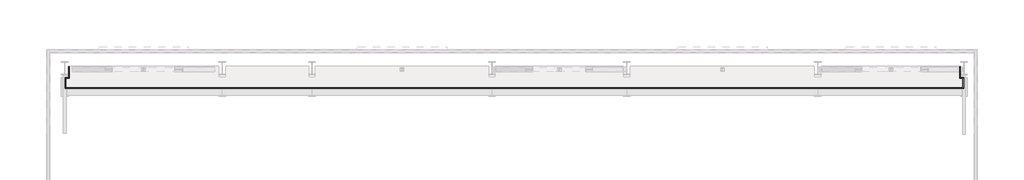
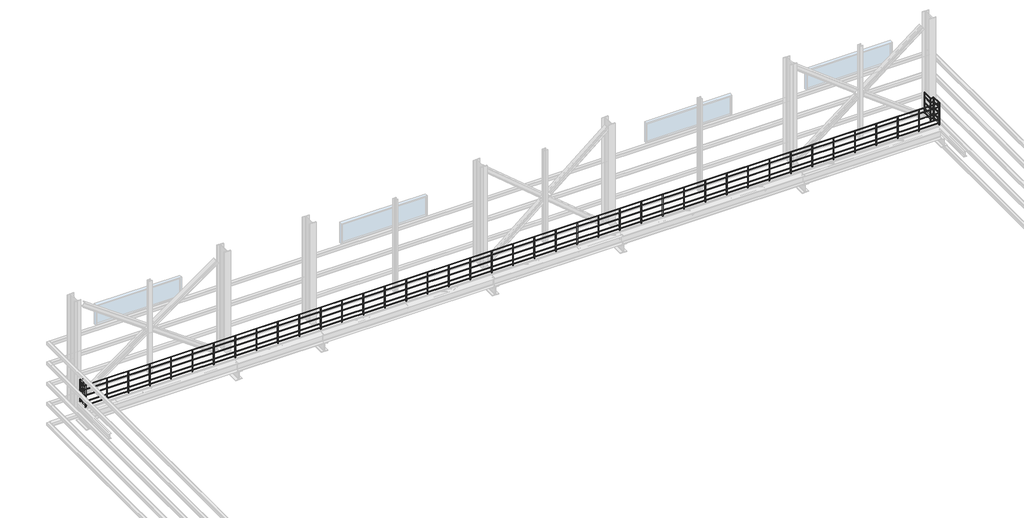
# One storey, part 4 of 4: 1 railing.
"""IFC4 building model written with IfcOpenShell, lengths in millimetres."""

from ifc_helpers import new_model, si_unit, frame, origin, place, context, project, spatial, polyline, circle_curve, ellipse_curve, outline, extrude, element, save
from ifc_brep_helpers import plane_surface, cylinder_surface, advanced_brep

model = new_model("IFC4")

# Units and contexts
model_context = context("Model", 3, world=origin())
ifc_project = project(units=[si_unit("LENGTHUNIT", "METRE", prefix="MILLI")], contexts=[model_context])

# Site, building, storey
site = spatial("IfcSite", under=ifc_project)
building = spatial("IfcBuilding", under=site)
storey = spatial("IfcBuildingStorey", under=building, Name="T.O.CRANE GIR.", Elevation=12299.9720055)

# Railing
placement = place(None, origin())
element("IfcRailing", 1, ObjectType="H_RL_AMH_Steel Handrail_H1100", at=placement, inside=storey, context=model_context, shape_type="SolidModel", body=[
    advanced_brep(
    [(165.0, 39119.5208589, 13466.9720055), (195.0, 39119.5208589, 13466.9720055), (165.0, 38634.5208589, 13466.9720055), (195.0, 38604.5208589, 13466.9720055), (15.0, 38634.5208589, 13466.9720055), (45.0, 38604.5208589, 13466.9720055), (15.0, 38164.5208589, 13466.9720055), (45.0, 38194.5208589, 13466.9720055), (39985.0, 38164.5208589, 13466.9720055), (39955.0, 38194.5208589, 13466.9720055), (39985.0, 38634.5208589, 13466.9720055), (39955.0, 38604.5208589, 13466.9720055), (39835.0, 38634.5208589, 13466.9720055), (39805.0, 38604.5208589, 13466.9720055), (39835.0, 39119.5208589, 13466.9720055), (39805.0, 39119.5208589, 13466.9720055)],
    [
        (0, 1, circle_curve(frame((180.0, 39119.5208589, 13466.9720055), z_axis=(0.0, 1.0, 0.0), x_axis=(1.0, 0.0, 0.0)), 15.0)),
        (1, 0, circle_curve(frame((180.0, 39119.5208589, 13466.9720055), z_axis=(0.0, 1.0, 0.0), x_axis=(1.0, 0.0, 0.0)), 15.0)),
        (0, 2),
        (2, 3, ellipse_curve(frame((180.0, 38619.5208589, 13466.9720055), z_axis=(0.707106781186548, 0.7071067811865469, 0.0), x_axis=(-0.7071067811865468, 0.7071067811865482, 0.0)), 21.2132034, 15.0)),
        (3, 1),
        (3, 2, ellipse_curve(frame((180.0, 38619.5208589, 13466.9720055), z_axis=(0.707106781186548, 0.7071067811865469, 0.0), x_axis=(-0.7071067811865468, 0.7071067811865482, 0.0)), 21.2132034, 15.0)),
        (2, 4),
        (4, 5, ellipse_curve(frame((30.0, 38619.5208589, 13466.9720055), z_axis=(0.707106781186548, 0.7071067811865469, 0.0), x_axis=(0.7071067811865472, -0.7071067811865479, 0.0)), 21.2132034, 15.0)),
        (5, 3),
        (5, 4, ellipse_curve(frame((30.0, 38619.5208589, 13466.9720055), z_axis=(0.707106781186548, 0.7071067811865469, 0.0), x_axis=(0.7071067811865472, -0.7071067811865479, 0.0)), 21.2132034, 15.0)),
        (4, 6),
        (6, 7, ellipse_curve(frame((30.0, 38179.5208589, 13466.9720055), z_axis=(-0.7071067811865459, 0.7071067811865491, 0.0), x_axis=(0.7071067811865491, 0.7071067811865458, 0.0)), 21.2132034, 15.0)),
        (7, 5),
        (7, 6, ellipse_curve(frame((30.0, 38179.5208589, 13466.9720055), z_axis=(-0.7071067811865459, 0.7071067811865491, 0.0), x_axis=(0.7071067811865491, 0.7071067811865458, 0.0)), 21.2132034, 15.0)),
        (6, 8),
        (8, 9, ellipse_curve(frame((39970.0, 38179.5208589, 13466.9720055), z_axis=(-0.7071067811865486, -0.7071067811865465, 0.0), x_axis=(-0.7071067811865465, 0.7071067811865486, 0.0)), 21.2132034, 15.0)),
        (9, 7),
        (9, 8, ellipse_curve(frame((39970.0, 38179.5208589, 13466.9720055), z_axis=(-0.7071067811865486, -0.7071067811865465, 0.0), x_axis=(-0.7071067811865465, 0.7071067811865486, 0.0)), 21.2132034, 15.0)),
        (8, 10),
        (10, 11, ellipse_curve(frame((39970.0, 38619.5208589, 13466.9720055), z_axis=(0.7071067811865476, -0.7071067811865474, 0.0), x_axis=(-0.7071067811865472, -0.7071067811865478, 0.0)), 21.2132034, 15.0)),
        (11, 9),
        (11, 10, ellipse_curve(frame((39970.0, 38619.5208589, 13466.9720055), z_axis=(0.7071067811865476, -0.7071067811865474, 0.0), x_axis=(-0.7071067811865472, -0.7071067811865478, 0.0)), 21.2132034, 15.0)),
        (10, 12),
        (12, 13, ellipse_curve(frame((39820.0, 38619.5208589, 13466.9720055), z_axis=(0.7071067811865476, -0.7071067811865474, 0.0), x_axis=(0.7071067811865475, 0.7071067811865475, 0.0)), 21.2132034, 15.0)),
        (13, 11),
        (13, 12, ellipse_curve(frame((39820.0, 38619.5208589, 13466.9720055), z_axis=(0.7071067811865476, -0.7071067811865474, 0.0), x_axis=(0.7071067811865475, 0.7071067811865475, 0.0)), 21.2132034, 15.0)),
        (14, 15, circle_curve(frame((39820.0, 39119.5208589, 13466.9720055), z_axis=(0.0, 1.0, 0.0), x_axis=(-1.0, 0.0, 0.0)), 15.0)),
        (15, 14, circle_curve(frame((39820.0, 39119.5208589, 13466.9720055), z_axis=(0.0, 1.0, 0.0), x_axis=(-1.0, 0.0, 0.0)), 15.0)),
        (12, 14),
        (15, 13),
    ],
    [
        plane_surface(frame((180.0, 39119.5208589, 13481.9720055), z_axis=(0.0, 1.0, 0.0), x_axis=(0.0, 0.0, -1.0))),
        cylinder_surface(frame((180.0, 39119.5208589, 13466.9720055), z_axis=(0.0, 1.0, 0.0), x_axis=(1.0, 0.0, 0.0)), 15.0),
        cylinder_surface(frame((180.0, 38619.5208589, 13466.9720055), z_axis=(1.0, 0.0, 0.0), x_axis=(0.0, -1.0, 0.0)), 15.0),
        cylinder_surface(frame((30.0, 38619.5208589, 13466.9720055), z_axis=(0.0, 1.0, 0.0), x_axis=(1.0, 0.0, 0.0)), 15.0),
        cylinder_surface(frame((30.0, 38179.5208589, 13466.9720055), z_axis=(-1.0, 0.0, 0.0), x_axis=(0.0, 1.0, 0.0)), 15.0),
        cylinder_surface(frame((39970.0, 38179.5208589, 13466.9720055), z_axis=(0.0, -1.0, 0.0), x_axis=(-1.0, 0.0, 0.0)), 15.0),
        cylinder_surface(frame((39970.0, 38619.5208589, 13466.9720055), z_axis=(1.0, 0.0, 0.0), x_axis=(0.0, -1.0, 0.0)), 15.0),
        plane_surface(frame((39820.0, 39119.5208589, 13481.9720055), z_axis=(0.0, 1.0, 0.0), x_axis=(0.0, 0.0, 1.0))),
        cylinder_surface(frame((39820.0, 38619.5208589, 13466.9720055), z_axis=(0.0, -1.0, 0.0), x_axis=(-1.0, 0.0, 0.0)), 15.0),
    ],
    [
        (0, [[1, 2]]),
        (1, [[-1, 3, 4, 5]]),
        (1, [[-2, -5, 6, -3]]),
        (2, [[-4, 7, 8, 9]]),
        (2, [[-6, -9, 10, -7]]),
        (3, [[-8, 11, 12, 13]]),
        (3, [[-10, -13, 14, -11]]),
        (4, [[-12, 15, 16, 17]]),
        (4, [[-14, -17, 18, -15]]),
        (5, [[-16, 19, 20, 21]]),
        (5, [[-18, -21, 22, -19]]),
        (6, [[-20, 23, 24, 25]]),
        (6, [[-22, -25, 26, -23]]),
        (7, [[27, 28]]),
        (8, [[-24, 29, -28, 30]]),
        (8, [[-26, -30, -27, -29]]),
    ],
),
    advanced_brep(
    [(15.0, 38634.5208589, 13266.9720055), (45.0, 38604.5208589, 13266.9720055), (45.0, 38194.5208589, 13266.9720055), (15.0, 38164.5208589, 13266.9720055), (39955.0, 38194.5208589, 13266.9720055), (39985.0, 38164.5208589, 13266.9720055), (39955.0, 38604.5208589, 13266.9720055), (39985.0, 38634.5208589, 13266.9720055), (39805.0, 38604.5208589, 13266.9720055), (39835.0, 38634.5208589, 13266.9720055), (39805.0, 39119.5208589, 13266.9720055), (39835.0, 39119.5208589, 13266.9720055), (195.0, 39119.5208589, 13266.9720055), (165.0, 39119.5208589, 13266.9720055), (195.0, 38604.5208589, 13266.9720055), (165.0, 38634.5208589, 13266.9720055)],
    [
        (0, 1, ellipse_curve(frame((30.0, 38619.5208589, 13266.9720055), z_axis=(-0.707106781186548, -0.7071067811865469, 0.0), x_axis=(-0.7071067811865467, 0.7071067811865482, 0.0)), 21.2132034, 15.0)),
        (1, 2),
        (2, 3, ellipse_curve(frame((30.0, 38179.5208589, 13266.9720055), z_axis=(-0.7071067811865459, 0.7071067811865491, 0.0), x_axis=(0.7071067811865491, 0.7071067811865458, 0.0)), 21.2132034, 15.0)),
        (3, 0),
        (1, 0, ellipse_curve(frame((30.0, 38619.5208589, 13266.9720055), z_axis=(-0.707106781186548, -0.7071067811865469, 0.0), x_axis=(-0.7071067811865467, 0.7071067811865482, 0.0)), 21.2132034, 15.0)),
        (3, 2, ellipse_curve(frame((30.0, 38179.5208589, 13266.9720055), z_axis=(-0.7071067811865459, 0.7071067811865491, 0.0), x_axis=(0.7071067811865491, 0.7071067811865458, 0.0)), 21.2132034, 15.0)),
        (2, 4),
        (4, 5, ellipse_curve(frame((39970.0, 38179.5208589, 13266.9720055), z_axis=(-0.7071067811865486, -0.7071067811865465, 0.0), x_axis=(-0.7071067811865465, 0.7071067811865486, 0.0)), 21.2132034, 15.0)),
        (5, 3),
        (5, 4, ellipse_curve(frame((39970.0, 38179.5208589, 13266.9720055), z_axis=(-0.7071067811865486, -0.7071067811865465, 0.0), x_axis=(-0.7071067811865465, 0.7071067811865486, 0.0)), 21.2132034, 15.0)),
        (4, 6),
        (6, 7, ellipse_curve(frame((39970.0, 38619.5208589, 13266.9720055), z_axis=(0.7071067811865476, -0.7071067811865474, 0.0), x_axis=(-0.7071067811865472, -0.7071067811865478, 0.0)), 21.2132034, 15.0)),
        (7, 5),
        (7, 6, ellipse_curve(frame((39970.0, 38619.5208589, 13266.9720055), z_axis=(0.7071067811865476, -0.7071067811865474, 0.0), x_axis=(-0.7071067811865472, -0.7071067811865478, 0.0)), 21.2132034, 15.0)),
        (6, 8),
        (8, 9, ellipse_curve(frame((39820.0, 38619.5208589, 13266.9720055), z_axis=(0.7071067811865476, -0.7071067811865474, 0.0), x_axis=(0.7071067811865475, 0.7071067811865475, 0.0)), 21.2132034, 15.0)),
        (9, 7),
        (9, 8, ellipse_curve(frame((39820.0, 38619.5208589, 13266.9720055), z_axis=(0.7071067811865476, -0.7071067811865474, 0.0), x_axis=(0.7071067811865475, 0.7071067811865475, 0.0)), 21.2132034, 15.0)),
        (10, 11, circle_curve(frame((39820.0, 39119.5208589, 13266.9720055), z_axis=(0.0, 1.0, 0.0), x_axis=(1.0, 0.0, 0.0)), 15.0)),
        (11, 10, circle_curve(frame((39820.0, 39119.5208589, 13266.9720055), z_axis=(0.0, 1.0, 0.0), x_axis=(1.0, 0.0, 0.0)), 15.0)),
        (8, 10),
        (11, 9),
        (12, 13, circle_curve(frame((180.0, 39119.5208589, 13266.9720055), z_axis=(0.0, 1.0, 0.0), x_axis=(-1.0, 0.0, 0.0)), 15.0)),
        (13, 12, circle_curve(frame((180.0, 39119.5208589, 13266.9720055), z_axis=(0.0, 1.0, 0.0), x_axis=(-1.0, 0.0, 0.0)), 15.0)),
        (12, 14),
        (14, 15, ellipse_curve(frame((180.0, 38619.5208589, 13266.9720055), z_axis=(0.707106781186548, 0.7071067811865469, 0.0), x_axis=(-0.7071067811865468, 0.7071067811865482, 0.0)), 21.2132034, 15.0)),
        (15, 13),
        (15, 14, ellipse_curve(frame((180.0, 38619.5208589, 13266.9720055), z_axis=(0.707106781186548, 0.7071067811865469, 0.0), x_axis=(-0.7071067811865468, 0.7071067811865482, 0.0)), 21.2132034, 15.0)),
        (14, 1),
        (0, 15),
    ],
    [
        cylinder_surface(frame((30.0, 38619.5208589, 13266.9720055), z_axis=(0.0, 1.0, 0.0), x_axis=(-1.0, 0.0, 0.0)), 15.0),
        cylinder_surface(frame((30.0, 38179.5208589, 13266.9720055), z_axis=(-1.0, 0.0, 0.0), x_axis=(0.0, -1.0, 0.0)), 15.0),
        cylinder_surface(frame((39970.0, 38179.5208589, 13266.9720055), z_axis=(0.0, -1.0, 0.0), x_axis=(1.0, 0.0, 0.0)), 15.0),
        cylinder_surface(frame((39970.0, 38619.5208589, 13266.9720055), z_axis=(1.0, 0.0, 0.0), x_axis=(0.0, 1.0, 0.0)), 15.0),
        plane_surface(frame((39820.0, 39119.5208589, 13281.9720055), z_axis=(0.0, 1.0, 0.0), x_axis=(0.0, 0.0, 1.0))),
        cylinder_surface(frame((39820.0, 38619.5208589, 13266.9720055), z_axis=(0.0, -1.0, 0.0), x_axis=(1.0, 0.0, 0.0)), 15.0),
        plane_surface(frame((180.0, 39119.5208589, 13281.9720055), z_axis=(0.0, 1.0, 0.0), x_axis=(0.0, 0.0, -1.0))),
        cylinder_surface(frame((180.0, 39119.5208589, 13266.9720055), z_axis=(0.0, 1.0, 0.0), x_axis=(-1.0, 0.0, 0.0)), 15.0),
        cylinder_surface(frame((180.0, 38619.5208589, 13266.9720055), z_axis=(1.0, 0.0, 0.0), x_axis=(0.0, 1.0, 0.0)), 15.0),
    ],
    [
        (0, [[1, 2, 3, 4]]),
        (0, [[5, -4, 6, -2]]),
        (1, [[-3, 7, 8, 9]]),
        (1, [[-6, -9, 10, -7]]),
        (2, [[-8, 11, 12, 13]]),
        (2, [[-10, -13, 14, -11]]),
        (3, [[-12, 15, 16, 17]]),
        (3, [[-14, -17, 18, -15]]),
        (4, [[19, 20]]),
        (5, [[-16, 21, -20, 22]]),
        (5, [[-18, -22, -19, -21]]),
        (6, [[23, 24]]),
        (7, [[-23, 25, 26, 27]]),
        (7, [[-24, -27, 28, -25]]),
        (8, [[-26, 29, -1, 30]]),
        (8, [[-28, -30, -5, -29]]),
    ],
),
    advanced_brep(
    [(15.0, 38634.5208589, 12966.9720055), (45.0, 38604.5208589, 12966.9720055), (45.0, 38194.5208589, 12966.9720055), (15.0, 38164.5208589, 12966.9720055), (39955.0, 38194.5208589, 12966.9720055), (39985.0, 38164.5208589, 12966.9720055), (39955.0, 38604.5208589, 12966.9720055), (39985.0, 38634.5208589, 12966.9720055), (39805.0, 38604.5208589, 12966.9720055), (39835.0, 38634.5208589, 12966.9720055), (39805.0, 39119.5208589, 12966.9720055), (39835.0, 39119.5208589, 12966.9720055), (195.0, 39119.5208589, 12966.9720055), (165.0, 39119.5208589, 12966.9720055), (195.0, 38604.5208589, 12966.9720055), (165.0, 38634.5208589, 12966.9720055)],
    [
        (0, 1, ellipse_curve(frame((30.0, 38619.5208589, 12966.9720055), z_axis=(-0.707106781186548, -0.7071067811865469, 0.0), x_axis=(-0.7071067811865467, 0.7071067811865482, 0.0)), 21.2132034, 15.0)),
        (1, 2),
        (2, 3, ellipse_curve(frame((30.0, 38179.5208589, 12966.9720055), z_axis=(-0.7071067811865459, 0.7071067811865491, 0.0), x_axis=(0.7071067811865491, 0.7071067811865458, 0.0)), 21.2132034, 15.0)),
        (3, 0),
        (1, 0, ellipse_curve(frame((30.0, 38619.5208589, 12966.9720055), z_axis=(-0.707106781186548, -0.7071067811865469, 0.0), x_axis=(-0.7071067811865467, 0.7071067811865482, 0.0)), 21.2132034, 15.0)),
        (3, 2, ellipse_curve(frame((30.0, 38179.5208589, 12966.9720055), z_axis=(-0.7071067811865459, 0.7071067811865491, 0.0), x_axis=(0.7071067811865491, 0.7071067811865458, 0.0)), 21.2132034, 15.0)),
        (2, 4),
        (4, 5, ellipse_curve(frame((39970.0, 38179.5208589, 12966.9720055), z_axis=(-0.7071067811865486, -0.7071067811865465, 0.0), x_axis=(-0.7071067811865465, 0.7071067811865486, 0.0)), 21.2132034, 15.0)),
        (5, 3),
        (5, 4, ellipse_curve(frame((39970.0, 38179.5208589, 12966.9720055), z_axis=(-0.7071067811865486, -0.7071067811865465, 0.0), x_axis=(-0.7071067811865465, 0.7071067811865486, 0.0)), 21.2132034, 15.0)),
        (4, 6),
        (6, 7, ellipse_curve(frame((39970.0, 38619.5208589, 12966.9720055), z_axis=(0.7071067811865476, -0.7071067811865474, 0.0), x_axis=(-0.7071067811865472, -0.7071067811865478, 0.0)), 21.2132034, 15.0)),
        (7, 5),
        (7, 6, ellipse_curve(frame((39970.0, 38619.5208589, 12966.9720055), z_axis=(0.7071067811865476, -0.7071067811865474, 0.0), x_axis=(-0.7071067811865472, -0.7071067811865478, 0.0)), 21.2132034, 15.0)),
        (6, 8),
        (8, 9, ellipse_curve(frame((39820.0, 38619.5208589, 12966.9720055), z_axis=(0.7071067811865476, -0.7071067811865474, 0.0), x_axis=(0.7071067811865475, 0.7071067811865475, 0.0)), 21.2132034, 15.0)),
        (9, 7),
        (9, 8, ellipse_curve(frame((39820.0, 38619.5208589, 12966.9720055), z_axis=(0.7071067811865476, -0.7071067811865474, 0.0), x_axis=(0.7071067811865475, 0.7071067811865475, 0.0)), 21.2132034, 15.0)),
        (10, 11, circle_curve(frame((39820.0, 39119.5208589, 12966.9720055), z_axis=(0.0, 1.0, 0.0), x_axis=(1.0, 0.0, 0.0)), 15.0)),
        (11, 10, circle_curve(frame((39820.0, 39119.5208589, 12966.9720055), z_axis=(0.0, 1.0, 0.0), x_axis=(1.0, 0.0, 0.0)), 15.0)),
        (8, 10),
        (11, 9),
        (12, 13, circle_curve(frame((180.0, 39119.5208589, 12966.9720055), z_axis=(0.0, 1.0, 0.0), x_axis=(-1.0, 0.0, 0.0)), 15.0)),
        (13, 12, circle_curve(frame((180.0, 39119.5208589, 12966.9720055), z_axis=(0.0, 1.0, 0.0), x_axis=(-1.0, 0.0, 0.0)), 15.0)),
        (12, 14),
        (14, 15, ellipse_curve(frame((180.0, 38619.5208589, 12966.9720055), z_axis=(0.707106781186548, 0.7071067811865469, 0.0), x_axis=(-0.7071067811865468, 0.7071067811865482, 0.0)), 21.2132034, 15.0)),
        (15, 13),
        (15, 14, ellipse_curve(frame((180.0, 38619.5208589, 12966.9720055), z_axis=(0.707106781186548, 0.7071067811865469, 0.0), x_axis=(-0.7071067811865468, 0.7071067811865482, 0.0)), 21.2132034, 15.0)),
        (14, 1),
        (0, 15),
    ],
    [
        cylinder_surface(frame((30.0, 38619.5208589, 12966.9720055), z_axis=(0.0, 1.0, 0.0), x_axis=(-1.0, 0.0, 0.0)), 15.0),
        cylinder_surface(frame((30.0, 38179.5208589, 12966.9720055), z_axis=(-1.0, 0.0, 0.0), x_axis=(0.0, -1.0, 0.0)), 15.0),
        cylinder_surface(frame((39970.0, 38179.5208589, 12966.9720055), z_axis=(0.0, -1.0, 0.0), x_axis=(1.0, 0.0, 0.0)), 15.0),
        cylinder_surface(frame((39970.0, 38619.5208589, 12966.9720055), z_axis=(1.0, 0.0, 0.0), x_axis=(0.0, 1.0, 0.0)), 15.0),
        plane_surface(frame((39820.0, 39119.5208589, 12981.9720055), z_axis=(0.0, 1.0, 0.0), x_axis=(0.0, 0.0, 1.0))),
        cylinder_surface(frame((39820.0, 38619.5208589, 12966.9720055), z_axis=(0.0, -1.0, 0.0), x_axis=(1.0, 0.0, 0.0)), 15.0),
        plane_surface(frame((180.0, 39119.5208589, 12981.9720055), z_axis=(0.0, 1.0, 0.0), x_axis=(0.0, 0.0, -1.0))),
        cylinder_surface(frame((180.0, 39119.5208589, 12966.9720055), z_axis=(0.0, 1.0, 0.0), x_axis=(-1.0, 0.0, 0.0)), 15.0),
        cylinder_surface(frame((180.0, 38619.5208589, 12966.9720055), z_axis=(1.0, 0.0, 0.0), x_axis=(0.0, 1.0, 0.0)), 15.0),
    ],
    [
        (0, [[1, 2, 3, 4]]),
        (0, [[5, -4, 6, -2]]),
        (1, [[-3, 7, 8, 9]]),
        (1, [[-6, -9, 10, -7]]),
        (2, [[-8, 11, 12, 13]]),
        (2, [[-10, -13, 14, -11]]),
        (3, [[-12, 15, 16, 17]]),
        (3, [[-14, -17, 18, -15]]),
        (4, [[19, 20]]),
        (5, [[-16, 21, -20, 22]]),
        (5, [[-18, -22, -19, -21]]),
        (6, [[23, 24]]),
        (7, [[-23, 25, 26, 27]]),
        (7, [[-24, -27, 28, -25]]),
        (8, [[-26, 29, -1, 30]]),
        (8, [[-28, -30, -5, -29]]),
    ],
),
    advanced_brep(
    [(195.0, 39119.5208589, 12666.9720055), (165.0, 39119.5208589, 12666.9720055), (195.0, 38604.5208589, 12666.9720055), (165.0, 38634.5208589, 12666.9720055), (45.0, 38604.5208589, 12666.9720055), (15.0, 38634.5208589, 12666.9720055), (45.0, 38194.5208589, 12666.9720055), (15.0, 38164.5208589, 12666.9720055), (39955.0, 38194.5208589, 12666.9720055), (39985.0, 38164.5208589, 12666.9720055), (39955.0, 38604.5208589, 12666.9720055), (39985.0, 38634.5208589, 12666.9720055), (39805.0, 38604.5208589, 12666.9720055), (39835.0, 38634.5208589, 12666.9720055), (39805.0, 39119.5208589, 12666.9720055), (39835.0, 39119.5208589, 12666.9720055)],
    [
        (0, 1, circle_curve(frame((180.0, 39119.5208589, 12666.9720055), z_axis=(0.0, 1.0, 0.0), x_axis=(-1.0, 0.0, 0.0)), 15.0)),
        (1, 0, circle_curve(frame((180.0, 39119.5208589, 12666.9720055), z_axis=(0.0, 1.0, 0.0), x_axis=(-1.0, 0.0, 0.0)), 15.0)),
        (0, 2),
        (2, 3, ellipse_curve(frame((180.0, 38619.5208589, 12666.9720055), z_axis=(0.707106781186548, 0.7071067811865469, 0.0), x_axis=(-0.7071067811865468, 0.7071067811865482, 0.0)), 21.2132034, 15.0)),
        (3, 1),
        (3, 2, ellipse_curve(frame((180.0, 38619.5208589, 12666.9720055), z_axis=(0.707106781186548, 0.7071067811865469, 0.0), x_axis=(-0.7071067811865468, 0.7071067811865482, 0.0)), 21.2132034, 15.0)),
        (2, 4),
        (4, 5, ellipse_curve(frame((30.0, 38619.5208589, 12666.9720055), z_axis=(0.707106781186548, 0.7071067811865469, 0.0), x_axis=(0.7071067811865472, -0.7071067811865479, 0.0)), 21.2132034, 15.0)),
        (5, 3),
        (5, 4, ellipse_curve(frame((30.0, 38619.5208589, 12666.9720055), z_axis=(0.707106781186548, 0.7071067811865469, 0.0), x_axis=(0.7071067811865472, -0.7071067811865479, 0.0)), 21.2132034, 15.0)),
        (4, 6),
        (6, 7, ellipse_curve(frame((30.0, 38179.5208589, 12666.9720055), z_axis=(-0.7071067811865459, 0.7071067811865491, 0.0), x_axis=(0.7071067811865491, 0.7071067811865458, 0.0)), 21.2132034, 15.0)),
        (7, 5),
        (7, 6, ellipse_curve(frame((30.0, 38179.5208589, 12666.9720055), z_axis=(-0.7071067811865459, 0.7071067811865491, 0.0), x_axis=(0.7071067811865491, 0.7071067811865458, 0.0)), 21.2132034, 15.0)),
        (6, 8),
        (8, 9, ellipse_curve(frame((39970.0, 38179.5208589, 12666.9720055), z_axis=(-0.7071067811865486, -0.7071067811865465, 0.0), x_axis=(-0.7071067811865465, 0.7071067811865486, 0.0)), 21.2132034, 15.0)),
        (9, 7),
        (9, 8, ellipse_curve(frame((39970.0, 38179.5208589, 12666.9720055), z_axis=(-0.7071067811865486, -0.7071067811865465, 0.0), x_axis=(-0.7071067811865465, 0.7071067811865486, 0.0)), 21.2132034, 15.0)),
        (8, 10),
        (10, 11, ellipse_curve(frame((39970.0, 38619.5208589, 12666.9720055), z_axis=(0.7071067811865476, -0.7071067811865474, 0.0), x_axis=(-0.7071067811865472, -0.7071067811865478, 0.0)), 21.2132034, 15.0)),
        (11, 9),
        (11, 10, ellipse_curve(frame((39970.0, 38619.5208589, 12666.9720055), z_axis=(0.7071067811865476, -0.7071067811865474, 0.0), x_axis=(-0.7071067811865472, -0.7071067811865478, 0.0)), 21.2132034, 15.0)),
        (10, 12),
        (12, 13, ellipse_curve(frame((39820.0, 38619.5208589, 12666.9720055), z_axis=(0.7071067811865476, -0.7071067811865474, 0.0), x_axis=(0.7071067811865475, 0.7071067811865475, 0.0)), 21.2132034, 15.0)),
        (13, 11),
        (13, 12, ellipse_curve(frame((39820.0, 38619.5208589, 12666.9720055), z_axis=(0.7071067811865476, -0.7071067811865474, 0.0), x_axis=(0.7071067811865475, 0.7071067811865475, 0.0)), 21.2132034, 15.0)),
        (14, 15, circle_curve(frame((39820.0, 39119.5208589, 12666.9720055), z_axis=(0.0, 1.0, 0.0), x_axis=(1.0, 0.0, 0.0)), 15.0)),
        (15, 14, circle_curve(frame((39820.0, 39119.5208589, 12666.9720055), z_axis=(0.0, 1.0, 0.0), x_axis=(1.0, 0.0, 0.0)), 15.0)),
        (12, 14),
        (15, 13),
    ],
    [
        plane_surface(frame((180.0, 39119.5208589, 12681.9720055), z_axis=(0.0, 1.0, 0.0), x_axis=(0.0, 0.0, -1.0))),
        cylinder_surface(frame((180.0, 39119.5208589, 12666.9720055), z_axis=(0.0, 1.0, 0.0), x_axis=(-1.0, 0.0, 0.0)), 15.0),
        cylinder_surface(frame((180.0, 38619.5208589, 12666.9720055), z_axis=(1.0, 0.0, 0.0), x_axis=(0.0, 1.0, 0.0)), 15.0),
        cylinder_surface(frame((30.0, 38619.5208589, 12666.9720055), z_axis=(0.0, 1.0, 0.0), x_axis=(-1.0, 0.0, 0.0)), 15.0),
        cylinder_surface(frame((30.0, 38179.5208589, 12666.9720055), z_axis=(-1.0, 0.0, 0.0), x_axis=(0.0, -1.0, 0.0)), 15.0),
        cylinder_surface(frame((39970.0, 38179.5208589, 12666.9720055), z_axis=(0.0, -1.0, 0.0), x_axis=(1.0, 0.0, 0.0)), 15.0),
        cylinder_surface(frame((39970.0, 38619.5208589, 12666.9720055), z_axis=(1.0, 0.0, 0.0), x_axis=(0.0, 1.0, 0.0)), 15.0),
        plane_surface(frame((39820.0, 39119.5208589, 12681.9720055), z_axis=(0.0, 1.0, 0.0), x_axis=(0.0, 0.0, 1.0))),
        cylinder_surface(frame((39820.0, 38619.5208589, 12666.9720055), z_axis=(0.0, -1.0, 0.0), x_axis=(1.0, 0.0, 0.0)), 15.0),
    ],
    [
        (0, [[1, 2]]),
        (1, [[-1, 3, 4, 5]]),
        (1, [[-2, -5, 6, -3]]),
        (2, [[-4, 7, 8, 9]]),
        (2, [[-6, -9, 10, -7]]),
        (3, [[-8, 11, 12, 13]]),
        (3, [[-10, -13, 14, -11]]),
        (4, [[-12, 15, 16, 17]]),
        (4, [[-14, -17, 18, -15]]),
        (5, [[-16, 19, 20, 21]]),
        (5, [[-18, -21, 22, -19]]),
        (6, [[-20, 23, 24, 25]]),
        (6, [[-22, -25, 26, -23]]),
        (7, [[27, 28]]),
        (8, [[-24, 29, -28, 30]]),
        (8, [[-26, -30, -27, -29]]),
    ],
),
    advanced_brep(
    [(195.0, 39119.5208589, 12466.9720055), (165.0, 39119.5208589, 12466.9720055), (195.0, 38604.5208589, 12466.9720055), (165.0, 38634.5208589, 12466.9720055), (45.0, 38604.5208589, 12466.9720055), (15.0, 38634.5208589, 12466.9720055), (45.0, 38194.5208589, 12466.9720055), (15.0, 38164.5208589, 12466.9720055), (39955.0, 38194.5208589, 12466.9720055), (39985.0, 38164.5208589, 12466.9720055), (39955.0, 38604.5208589, 12466.9720055), (39985.0, 38634.5208589, 12466.9720055), (39805.0, 38604.5208589, 12466.9720055), (39835.0, 38634.5208589, 12466.9720055), (39805.0, 39119.5208589, 12466.9720055), (39835.0, 39119.5208589, 12466.9720055)],
    [
        (0, 1, circle_curve(frame((180.0, 39119.5208589, 12466.9720055), z_axis=(0.0, 1.0, 0.0), x_axis=(-1.0, 0.0, 0.0)), 15.0)),
        (1, 0, circle_curve(frame((180.0, 39119.5208589, 12466.9720055), z_axis=(0.0, 1.0, 0.0), x_axis=(-1.0, 0.0, 0.0)), 15.0)),
        (0, 2),
        (2, 3, ellipse_curve(frame((180.0, 38619.5208589, 12466.9720055), z_axis=(0.707106781186548, 0.7071067811865469, 0.0), x_axis=(-0.7071067811865468, 0.7071067811865482, 0.0)), 21.2132034, 15.0)),
        (3, 1),
        (3, 2, ellipse_curve(frame((180.0, 38619.5208589, 12466.9720055), z_axis=(0.707106781186548, 0.7071067811865469, 0.0), x_axis=(-0.7071067811865468, 0.7071067811865482, 0.0)), 21.2132034, 15.0)),
        (2, 4),
        (4, 5, ellipse_curve(frame((30.0, 38619.5208589, 12466.9720055), z_axis=(0.707106781186548, 0.7071067811865469, 0.0), x_axis=(0.7071067811865472, -0.7071067811865479, 0.0)), 21.2132034, 15.0)),
        (5, 3),
        (5, 4, ellipse_curve(frame((30.0, 38619.5208589, 12466.9720055), z_axis=(0.707106781186548, 0.7071067811865469, 0.0), x_axis=(0.7071067811865472, -0.7071067811865479, 0.0)), 21.2132034, 15.0)),
        (4, 6),
        (6, 7, ellipse_curve(frame((30.0, 38179.5208589, 12466.9720055), z_axis=(-0.7071067811865459, 0.7071067811865491, 0.0), x_axis=(0.7071067811865491, 0.7071067811865458, 0.0)), 21.2132034, 15.0)),
        (7, 5),
        (7, 6, ellipse_curve(frame((30.0, 38179.5208589, 12466.9720055), z_axis=(-0.7071067811865459, 0.7071067811865491, 0.0), x_axis=(0.7071067811865491, 0.7071067811865458, 0.0)), 21.2132034, 15.0)),
        (6, 8),
        (8, 9, ellipse_curve(frame((39970.0, 38179.5208589, 12466.9720055), z_axis=(-0.7071067811865486, -0.7071067811865465, 0.0), x_axis=(-0.7071067811865465, 0.7071067811865486, 0.0)), 21.2132034, 15.0)),
        (9, 7),
        (9, 8, ellipse_curve(frame((39970.0, 38179.5208589, 12466.9720055), z_axis=(-0.7071067811865486, -0.7071067811865465, 0.0), x_axis=(-0.7071067811865465, 0.7071067811865486, 0.0)), 21.2132034, 15.0)),
        (8, 10),
        (10, 11, ellipse_curve(frame((39970.0, 38619.5208589, 12466.9720055), z_axis=(0.7071067811865476, -0.7071067811865474, 0.0), x_axis=(-0.7071067811865472, -0.7071067811865478, 0.0)), 21.2132034, 15.0)),
        (11, 9),
        (11, 10, ellipse_curve(frame((39970.0, 38619.5208589, 12466.9720055), z_axis=(0.7071067811865476, -0.7071067811865474, 0.0), x_axis=(-0.7071067811865472, -0.7071067811865478, 0.0)), 21.2132034, 15.0)),
        (10, 12),
        (12, 13, ellipse_curve(frame((39820.0, 38619.5208589, 12466.9720055), z_axis=(0.7071067811865476, -0.7071067811865474, 0.0), x_axis=(0.7071067811865475, 0.7071067811865475, 0.0)), 21.2132034, 15.0)),
        (13, 11),
        (13, 12, ellipse_curve(frame((39820.0, 38619.5208589, 12466.9720055), z_axis=(0.7071067811865476, -0.7071067811865474, 0.0), x_axis=(0.7071067811865475, 0.7071067811865475, 0.0)), 21.2132034, 15.0)),
        (14, 15, circle_curve(frame((39820.0, 39119.5208589, 12466.9720055), z_axis=(0.0, 1.0, 0.0), x_axis=(1.0, 0.0, 0.0)), 15.0)),
        (15, 14, circle_curve(frame((39820.0, 39119.5208589, 12466.9720055), z_axis=(0.0, 1.0, 0.0), x_axis=(1.0, 0.0, 0.0)), 15.0)),
        (12, 14),
        (15, 13),
    ],
    [
        plane_surface(frame((180.0, 39119.5208589, 12481.9720055), z_axis=(0.0, 1.0, 0.0), x_axis=(0.0, 0.0, -1.0))),
        cylinder_surface(frame((180.0, 39119.5208589, 12466.9720055), z_axis=(0.0, 1.0, 0.0), x_axis=(-1.0, 0.0, 0.0)), 15.0),
        cylinder_surface(frame((180.0, 38619.5208589, 12466.9720055), z_axis=(1.0, 0.0, 0.0), x_axis=(0.0, 1.0, 0.0)), 15.0),
        cylinder_surface(frame((30.0, 38619.5208589, 12466.9720055), z_axis=(0.0, 1.0, 0.0), x_axis=(-1.0, 0.0, 0.0)), 15.0),
        cylinder_surface(frame((30.0, 38179.5208589, 12466.9720055), z_axis=(-1.0, 0.0, 0.0), x_axis=(0.0, -1.0, 0.0)), 15.0),
        cylinder_surface(frame((39970.0, 38179.5208589, 12466.9720055), z_axis=(0.0, -1.0, 0.0), x_axis=(1.0, 0.0, 0.0)), 15.0),
        cylinder_surface(frame((39970.0, 38619.5208589, 12466.9720055), z_axis=(1.0, 0.0, 0.0), x_axis=(0.0, 1.0, 0.0)), 15.0),
        plane_surface(frame((39820.0, 39119.5208589, 12481.9720055), z_axis=(0.0, 1.0, 0.0), x_axis=(0.0, 0.0, 1.0))),
        cylinder_surface(frame((39820.0, 38619.5208589, 12466.9720055), z_axis=(0.0, -1.0, 0.0), x_axis=(1.0, 0.0, 0.0)), 15.0),
    ],
    [
        (0, [[1, 2]]),
        (1, [[-1, 3, 4, 5]]),
        (1, [[-2, -5, 6, -3]]),
        (2, [[-4, 7, 8, 9]]),
        (2, [[-6, -9, 10, -7]]),
        (3, [[-8, 11, 12, 13]]),
        (3, [[-10, -13, 14, -11]]),
        (4, [[-12, 15, 16, 17]]),
        (4, [[-14, -17, 18, -15]]),
        (5, [[-16, 19, 20, 21]]),
        (5, [[-18, -21, 22, -19]]),
        (6, [[-20, 23, 24, 25]]),
        (6, [[-22, -25, 26, -23]]),
        (7, [[27, 28]]),
        (8, [[-24, 29, -28, 30]]),
        (8, [[-26, -30, -27, -29]]),
    ],
),
    extrude(outline(polyline([(39017.5, 38167.0208589), (39017.5, 38192.0208589), (39042.5, 38192.0208589), (39042.5, 38167.0208589), (39017.5, 38167.0208589)])), frame((0.0, 0.0, 12381.9720055), z_axis=(0.0, 0.0, 1.0), x_axis=(1.0, 0.0, 0.0)), (0.0, 0.0, 1.0), 1070.0),
    extrude(outline(polyline([(38017.5, 38167.0208589), (38017.5, 38192.0208589), (38042.5, 38192.0208589), (38042.5, 38167.0208589), (38017.5, 38167.0208589)])), frame((0.0, 0.0, 12381.9720055), z_axis=(0.0, 0.0, 1.0), x_axis=(1.0, 0.0, 0.0)), (0.0, 0.0, 1.0), 1070.0),
    extrude(outline(polyline([(37017.5, 38167.0208589), (37017.5, 38192.0208589), (37042.5, 38192.0208589), (37042.5, 38167.0208589), (37017.5, 38167.0208589)])), frame((0.0, 0.0, 12381.9720055), z_axis=(0.0, 0.0, 1.0), x_axis=(1.0, 0.0, 0.0)), (0.0, 0.0, 1.0), 1070.0),
    extrude(outline(polyline([(36017.5, 38167.0208589), (36017.5, 38192.0208589), (36042.5, 38192.0208589), (36042.5, 38167.0208589), (36017.5, 38167.0208589)])), frame((0.0, 0.0, 12381.9720055), z_axis=(0.0, 0.0, 1.0), x_axis=(1.0, 0.0, 0.0)), (0.0, 0.0, 1.0), 1070.0),
    extrude(outline(polyline([(35017.5, 38167.0208589), (35017.5, 38192.0208589), (35042.5, 38192.0208589), (35042.5, 38167.0208589), (35017.5, 38167.0208589)])), frame((0.0, 0.0, 12381.9720055), z_axis=(0.0, 0.0, 1.0), x_axis=(1.0, 0.0, 0.0)), (0.0, 0.0, 1.0), 1070.0),
    extrude(outline(polyline([(34017.5, 38167.0208589), (34017.5, 38192.0208589), (34042.5, 38192.0208589), (34042.5, 38167.0208589), (34017.5, 38167.0208589)])), frame((0.0, 0.0, 12381.9720055), z_axis=(0.0, 0.0, 1.0), x_axis=(1.0, 0.0, 0.0)), (0.0, 0.0, 1.0), 1070.0),
    extrude(outline(polyline([(33017.5, 38167.0208589), (33017.5, 38192.0208589), (33042.5, 38192.0208589), (33042.5, 38167.0208589), (33017.5, 38167.0208589)])), frame((0.0, 0.0, 12381.9720055), z_axis=(0.0, 0.0, 1.0), x_axis=(1.0, 0.0, 0.0)), (0.0, 0.0, 1.0), 1070.0),
    extrude(outline(polyline([(32017.5, 38167.0208589), (32017.5, 38192.0208589), (32042.5, 38192.0208589), (32042.5, 38167.0208589), (32017.5, 38167.0208589)])), frame((0.0, 0.0, 12381.9720055), z_axis=(0.0, 0.0, 1.0), x_axis=(1.0, 0.0, 0.0)), (0.0, 0.0, 1.0), 1070.0),
    extrude(outline(polyline([(31017.5, 38167.0208589), (31017.5, 38192.0208589), (31042.5, 38192.0208589), (31042.5, 38167.0208589), (31017.5, 38167.0208589)])), frame((0.0, 0.0, 12381.9720055), z_axis=(0.0, 0.0, 1.0), x_axis=(1.0, 0.0, 0.0)), (0.0, 0.0, 1.0), 1070.0),
    extrude(outline(polyline([(30017.5, 38167.0208589), (30017.5, 38192.0208589), (30042.5, 38192.0208589), (30042.5, 38167.0208589), (30017.5, 38167.0208589)])), frame((0.0, 0.0, 12381.9720055), z_axis=(0.0, 0.0, 1.0), x_axis=(1.0, 0.0, 0.0)), (0.0, 0.0, 1.0), 1070.0),
    extrude(outline(polyline([(29017.5, 38167.0208589), (29017.5, 38192.0208589), (29042.5, 38192.0208589), (29042.5, 38167.0208589), (29017.5, 38167.0208589)])), frame((0.0, 0.0, 12381.9720055), z_axis=(0.0, 0.0, 1.0), x_axis=(1.0, 0.0, 0.0)), (0.0, 0.0, 1.0), 1070.0),
    extrude(outline(polyline([(28017.5, 38167.0208589), (28017.5, 38192.0208589), (28042.5, 38192.0208589), (28042.5, 38167.0208589), (28017.5, 38167.0208589)])), frame((0.0, 0.0, 12381.9720055), z_axis=(0.0, 0.0, 1.0), x_axis=(1.0, 0.0, 0.0)), (0.0, 0.0, 1.0), 1070.0),
    extrude(outline(polyline([(27017.5, 38167.0208589), (27017.5, 38192.0208589), (27042.5, 38192.0208589), (27042.5, 38167.0208589), (27017.5, 38167.0208589)])), frame((0.0, 0.0, 12381.9720055), z_axis=(0.0, 0.0, 1.0), x_axis=(1.0, 0.0, 0.0)), (0.0, 0.0, 1.0), 1070.0),
    extrude(outline(polyline([(26017.5, 38167.0208589), (26017.5, 38192.0208589), (26042.5, 38192.0208589), (26042.5, 38167.0208589), (26017.5, 38167.0208589)])), frame((0.0, 0.0, 12381.9720055), z_axis=(0.0, 0.0, 1.0), x_axis=(1.0, 0.0, 0.0)), (0.0, 0.0, 1.0), 1070.0),
    extrude(outline(polyline([(25017.5, 38167.0208589), (25017.5, 38192.0208589), (25042.5, 38192.0208589), (25042.5, 38167.0208589), (25017.5, 38167.0208589)])), frame((0.0, 0.0, 12381.9720055), z_axis=(0.0, 0.0, 1.0), x_axis=(1.0, 0.0, 0.0)), (0.0, 0.0, 1.0), 1070.0),
    extrude(outline(polyline([(24017.5, 38167.0208589), (24017.5, 38192.0208589), (24042.5, 38192.0208589), (24042.5, 38167.0208589), (24017.5, 38167.0208589)])), frame((0.0, 0.0, 12381.9720055), z_axis=(0.0, 0.0, 1.0), x_axis=(1.0, 0.0, 0.0)), (0.0, 0.0, 1.0), 1070.0),
    extrude(outline(polyline([(23017.5, 38167.0208589), (23017.5, 38192.0208589), (23042.5, 38192.0208589), (23042.5, 38167.0208589), (23017.5, 38167.0208589)])), frame((0.0, 0.0, 12381.9720055), z_axis=(0.0, 0.0, 1.0), x_axis=(1.0, 0.0, 0.0)), (0.0, 0.0, 1.0), 1070.0),
    extrude(outline(polyline([(22017.5, 38167.0208589), (22017.5, 38192.0208589), (22042.5, 38192.0208589), (22042.5, 38167.0208589), (22017.5, 38167.0208589)])), frame((0.0, 0.0, 12381.9720055), z_axis=(0.0, 0.0, 1.0), x_axis=(1.0, 0.0, 0.0)), (0.0, 0.0, 1.0), 1070.0),
    extrude(outline(polyline([(21017.5, 38167.0208589), (21017.5, 38192.0208589), (21042.5, 38192.0208589), (21042.5, 38167.0208589), (21017.5, 38167.0208589)])), frame((0.0, 0.0, 12381.9720055), z_axis=(0.0, 0.0, 1.0), x_axis=(1.0, 0.0, 0.0)), (0.0, 0.0, 1.0), 1070.0),
    extrude(outline(polyline([(20017.5, 38167.0208589), (20017.5, 38192.0208589), (20042.5, 38192.0208589), (20042.5, 38167.0208589), (20017.5, 38167.0208589)])), frame((0.0, 0.0, 12381.9720055), z_axis=(0.0, 0.0, 1.0), x_axis=(1.0, 0.0, 0.0)), (0.0, 0.0, 1.0), 1070.0),
    extrude(outline(polyline([(19017.5, 38167.0208589), (19017.5, 38192.0208589), (19042.5, 38192.0208589), (19042.5, 38167.0208589), (19017.5, 38167.0208589)])), frame((0.0, 0.0, 12381.9720055), z_axis=(0.0, 0.0, 1.0), x_axis=(1.0, 0.0, 0.0)), (0.0, 0.0, 1.0), 1070.0),
    extrude(outline(polyline([(18017.5, 38167.0208589), (18017.5, 38192.0208589), (18042.5, 38192.0208589), (18042.5, 38167.0208589), (18017.5, 38167.0208589)])), frame((0.0, 0.0, 12381.9720055), z_axis=(0.0, 0.0, 1.0), x_axis=(1.0, 0.0, 0.0)), (0.0, 0.0, 1.0), 1070.0),
    extrude(outline(polyline([(17017.5, 38167.0208589), (17017.5, 38192.0208589), (17042.5, 38192.0208589), (17042.5, 38167.0208589), (17017.5, 38167.0208589)])), frame((0.0, 0.0, 12381.9720055), z_axis=(0.0, 0.0, 1.0), x_axis=(1.0, 0.0, 0.0)), (0.0, 0.0, 1.0), 1070.0),
    extrude(outline(polyline([(16017.5, 38167.0208589), (16017.5, 38192.0208589), (16042.5, 38192.0208589), (16042.5, 38167.0208589), (16017.5, 38167.0208589)])), frame((0.0, 0.0, 12381.9720055), z_axis=(0.0, 0.0, 1.0), x_axis=(1.0, 0.0, 0.0)), (0.0, 0.0, 1.0), 1070.0),
    extrude(outline(polyline([(15017.5, 38167.0208589), (15017.5, 38192.0208589), (15042.5, 38192.0208589), (15042.5, 38167.0208589), (15017.5, 38167.0208589)])), frame((0.0, 0.0, 12381.9720055), z_axis=(0.0, 0.0, 1.0), x_axis=(1.0, 0.0, 0.0)), (0.0, 0.0, 1.0), 1070.0),
    extrude(outline(polyline([(14017.5, 38167.0208589), (14017.5, 38192.0208589), (14042.5, 38192.0208589), (14042.5, 38167.0208589), (14017.5, 38167.0208589)])), frame((0.0, 0.0, 12381.9720055), z_axis=(0.0, 0.0, 1.0), x_axis=(1.0, 0.0, 0.0)), (0.0, 0.0, 1.0), 1070.0),
    extrude(outline(polyline([(13017.5, 38167.0208589), (13017.5, 38192.0208589), (13042.5, 38192.0208589), (13042.5, 38167.0208589), (13017.5, 38167.0208589)])), frame((0.0, 0.0, 12381.9720055), z_axis=(0.0, 0.0, 1.0), x_axis=(1.0, 0.0, 0.0)), (0.0, 0.0, 1.0), 1070.0),
    extrude(outline(polyline([(12017.5, 38167.0208589), (12017.5, 38192.0208589), (12042.5, 38192.0208589), (12042.5, 38167.0208589), (12017.5, 38167.0208589)])), frame((0.0, 0.0, 12381.9720055), z_axis=(0.0, 0.0, 1.0), x_axis=(1.0, 0.0, 0.0)), (0.0, 0.0, 1.0), 1070.0),
    extrude(outline(polyline([(11017.5, 38167.0208589), (11017.5, 38192.0208589), (11042.5, 38192.0208589), (11042.5, 38167.0208589), (11017.5, 38167.0208589)])), frame((0.0, 0.0, 12381.9720055), z_axis=(0.0, 0.0, 1.0), x_axis=(1.0, 0.0, 0.0)), (0.0, 0.0, 1.0), 1070.0),
    extrude(outline(polyline([(10017.5, 38167.0208589), (10017.5, 38192.0208589), (10042.5, 38192.0208589), (10042.5, 38167.0208589), (10017.5, 38167.0208589)])), frame((0.0, 0.0, 12381.9720055), z_axis=(0.0, 0.0, 1.0), x_axis=(1.0, 0.0, 0.0)), (0.0, 0.0, 1.0), 1070.0),
    extrude(outline(polyline([(9017.5, 38167.0208589), (9017.5, 38192.0208589), (9042.5, 38192.0208589), (9042.5, 38167.0208589), (9017.5, 38167.0208589)])), frame((0.0, 0.0, 12381.9720055), z_axis=(0.0, 0.0, 1.0), x_axis=(1.0, 0.0, 0.0)), (0.0, 0.0, 1.0), 1070.0),
    extrude(outline(polyline([(8017.5, 38167.0208589), (8017.5, 38192.0208589), (8042.5, 38192.0208589), (8042.5, 38167.0208589), (8017.5, 38167.0208589)])), frame((0.0, 0.0, 12381.9720055), z_axis=(0.0, 0.0, 1.0), x_axis=(1.0, 0.0, 0.0)), (0.0, 0.0, 1.0), 1070.0),
    extrude(outline(polyline([(7017.5, 38167.0208589), (7017.5, 38192.0208589), (7042.5, 38192.0208589), (7042.5, 38167.0208589), (7017.5, 38167.0208589)])), frame((0.0, 0.0, 12381.9720055), z_axis=(0.0, 0.0, 1.0), x_axis=(1.0, 0.0, 0.0)), (0.0, 0.0, 1.0), 1070.0),
    extrude(outline(polyline([(6017.5, 38167.0208589), (6017.5, 38192.0208589), (6042.5, 38192.0208589), (6042.5, 38167.0208589), (6017.5, 38167.0208589)])), frame((0.0, 0.0, 12381.9720055), z_axis=(0.0, 0.0, 1.0), x_axis=(1.0, 0.0, 0.0)), (0.0, 0.0, 1.0), 1070.0),
    extrude(outline(polyline([(5017.5, 38167.0208589), (5017.5, 38192.0208589), (5042.5, 38192.0208589), (5042.5, 38167.0208589), (5017.5, 38167.0208589)])), frame((0.0, 0.0, 12381.9720055), z_axis=(0.0, 0.0, 1.0), x_axis=(1.0, 0.0, 0.0)), (0.0, 0.0, 1.0), 1070.0),
    extrude(outline(polyline([(4017.5, 38167.0208589), (4017.5, 38192.0208589), (4042.5, 38192.0208589), (4042.5, 38167.0208589), (4017.5, 38167.0208589)])), frame((0.0, 0.0, 12381.9720055), z_axis=(0.0, 0.0, 1.0), x_axis=(1.0, 0.0, 0.0)), (0.0, 0.0, 1.0), 1070.0),
    extrude(outline(polyline([(3017.5, 38167.0208589), (3017.5, 38192.0208589), (3042.5, 38192.0208589), (3042.5, 38167.0208589), (3017.5, 38167.0208589)])), frame((0.0, 0.0, 12381.9720055), z_axis=(0.0, 0.0, 1.0), x_axis=(1.0, 0.0, 0.0)), (0.0, 0.0, 1.0), 1070.0),
    extrude(outline(polyline([(2017.5, 38167.0208589), (2017.5, 38192.0208589), (2042.5, 38192.0208589), (2042.5, 38167.0208589), (2017.5, 38167.0208589)])), frame((0.0, 0.0, 12381.9720055), z_axis=(0.0, 0.0, 1.0), x_axis=(1.0, 0.0, 0.0)), (0.0, 0.0, 1.0), 1070.0),
    extrude(outline(polyline([(1017.5, 38167.0208589), (1017.5, 38192.0208589), (1042.5, 38192.0208589), (1042.5, 38167.0208589), (1017.5, 38167.0208589)])), frame((0.0, 0.0, 12381.9720055), z_axis=(0.0, 0.0, 1.0), x_axis=(1.0, 0.0, 0.0)), (0.0, 0.0, 1.0), 1070.0),
    extrude(outline(polyline([(39832.5, 38632.0208589), (39832.5, 38607.0208589), (39807.5, 38607.0208589), (39807.5, 38632.0208589), (39832.5, 38632.0208589)])), frame((0.0, 0.0, 12381.9720055), z_axis=(0.0, 0.0, 1.0), x_axis=(1.0, 0.0, 0.0)), (0.0, 0.0, 1.0), 1070.0),
    extrude(outline(polyline([(39982.5, 38607.0208589), (39957.5, 38607.0208589), (39957.5, 38632.0208589), (39982.5, 38632.0208589), (39982.5, 38607.0208589)])), frame((0.0, 0.0, 12381.9720055), z_axis=(0.0, 0.0, 1.0), x_axis=(1.0, 0.0, 0.0)), (0.0, 0.0, 1.0), 1070.0),
    extrude(outline(polyline([(39957.5, 38167.0208589), (39957.5, 38192.0208589), (39982.5, 38192.0208589), (39982.5, 38167.0208589), (39957.5, 38167.0208589)])), frame((0.0, 0.0, 12381.9720055), z_axis=(0.0, 0.0, 1.0), x_axis=(1.0, 0.0, 0.0)), (0.0, 0.0, 1.0), 1070.0),
    extrude(outline(polyline([(17.5, 38192.0208589), (42.5, 38192.0208589), (42.5, 38167.0208589), (17.5, 38167.0208589), (17.5, 38192.0208589)])), frame((0.0, 0.0, 12381.9720055), z_axis=(0.0, 0.0, 1.0), x_axis=(1.0, 0.0, 0.0)), (0.0, 0.0, 1.0), 1070.0),
    extrude(outline(polyline([(42.5, 38632.0208589), (42.5, 38607.0208589), (17.5, 38607.0208589), (17.5, 38632.0208589), (42.5, 38632.0208589)])), frame((0.0, 0.0, 12381.9720055), z_axis=(0.0, 0.0, 1.0), x_axis=(1.0, 0.0, 0.0)), (0.0, 0.0, 1.0), 1070.0),
    extrude(outline(polyline([(167.5, 38632.0208589), (192.5, 38632.0208589), (192.5, 38607.0208589), (167.5, 38607.0208589), (167.5, 38632.0208589)])), frame((0.0, 0.0, 12381.9720055), z_axis=(0.0, 0.0, 1.0), x_axis=(1.0, 0.0, 0.0)), (0.0, 0.0, 1.0), 1070.0),
    extrude(outline(polyline([(39832.5, 39094.5208589), (39807.5, 39094.5208589), (39807.5, 39119.5208589), (39832.5, 39119.5208589), (39832.5, 39094.5208589)])), frame((0.0, 0.0, 12381.9720055), z_axis=(0.0, 0.0, 1.0), x_axis=(1.0, 0.0, 0.0)), (0.0, 0.0, 1.0), 1070.0),
    extrude(outline(polyline([(167.5, 39119.5208589), (192.5, 39119.5208589), (192.5, 39094.5208589), (167.5, 39094.5208589), (167.5, 39119.5208589)])), frame((0.0, 0.0, 12381.9720055), z_axis=(0.0, 0.0, 1.0), x_axis=(1.0, 0.0, 0.0)), (0.0, 0.0, 1.0), 1070.0),
])

save(model, "model.ifc")

# Revit data of these elements
# Type "H_RL_AMH_Steel Handrail_H1100"
#   Description = "HANDRAIL"
#   Type Mark = "SH"
#   H_WM Code_1 = "S02AA020-00001 | Miscellaneous Steel Fabrication Work | Shelter/Building | Steel Handrails | Material: (   ) | H=(  )mm"
#   H_WM Code_2 = "S04AA020-00001 | Miscellaneous Steel Erection Work | Shelter/Building | Steel Handrails | Material: (   ) | H=(  )mm"
#   H_Q'ty Cal Type Tag = "RL-Q1"
#   built-in parameter 1008612 = 0.019685 (stored number, unit not read)
#   built-in parameter 1008611 = 0.0984252 (stored number, unit not read)
#   built-in parameter 1008609 = 3.28084 (stored number, unit not read)
#   built-in parameter 1008604 = 0.19685 (stored number, unit not read)
#   built-in parameter 1008603 = 0.164042 (stored number, unit not read)
#   Railing Height = 1.1000 m
#   built-in parameter 1008630 = 2
#   built-in parameter 1008610 = 1
#   built-in parameter 1008605 = 1
#   built-in parameter 1008618 = 난간동자 - 정사각형1 : 25mm
# Element 1 (IfcRailing, "H_RL_AMH_Steel Handrail_H1100")
#   built-in parameter 1008621 = 0.269029 (stored number, unit not read)
#   Phase Created = New Construction
#   Materials on its faces: "S02AA020-00001_Steel handrails"
# Materials
#   "S02AA020-00001_Steel handrails": class "Metal", colour RGB 120 120 120, transparency 0, Comments = "(30KG/M>Weight)", Description = "Structural steel 50ksi", Cost = 0
